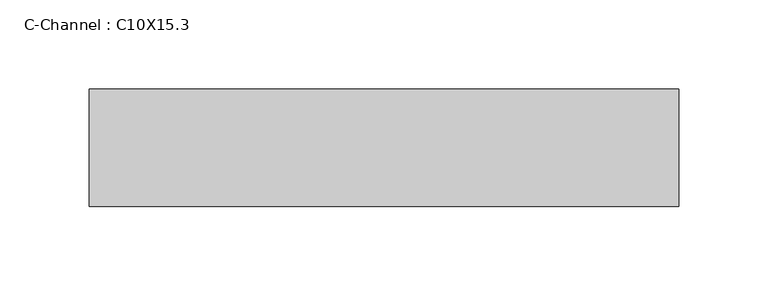
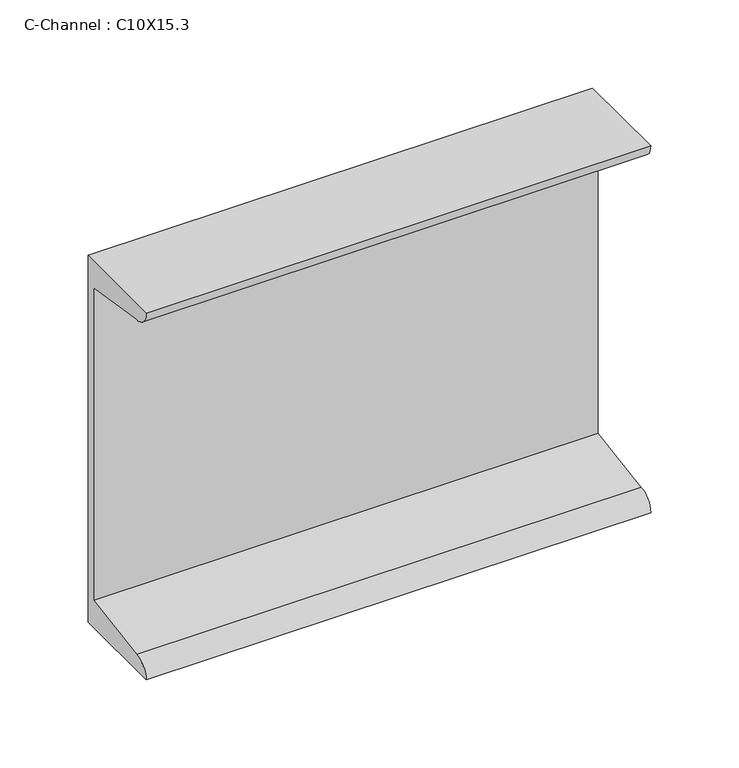
"""IFC4 building model written with IfcOpenShell, lengths in millimetres: beam geometry, C-Channel : C10X15.3."""

from ifc_helpers import new_model, si_unit, point, frame, frame_2d, origin, place, context, project, spatial, polyline, circle_curve, trimmed, segment, composite_curve, outline, extrude, source, transform, mapped, element, save


def c_channel_c10x15_3_927e855d(model_context):
    return source(origin(), model_context, "Body", "SweptSolid", [
        extrude(outline(composite_curve([segment(polyline([(16.1036, 127.0), (16.1036, -127.0), (-49.9364, -127.0)]), True, "CONTINUOUS"), segment(trimmed(circle_curve(frame_2d((-38.862, -127.0)), 11.0744), [point((-49.9364, -127.0))], [point((-38.862, -115.9256))], False, "CARTESIAN"), True, "CONTINUOUS"), segment(polyline([(-38.862, -115.9256), (10.0076, -108.1854158), (10.0076, 108.1854158), (-38.862, 115.9256)]), True, "CONTINUOUS"), segment(trimmed(circle_curve(frame_2d((-38.862, 127.0)), 11.0744), [point((-38.862, 115.9256))], [point((-49.9364, 127.0))], False, "CARTESIAN"), True, "CONTINUOUS"), segment(polyline([(-49.9364, 127.0), (16.1036, 127.0)]), True, "CONTINUOUS")], self_intersect=False)), frame((-178.308, 0.0, 0.0), z_axis=(1.0, 0.0, 0.0), x_axis=(0.0, 1.0, 0.0)), (0.0, 0.0, 1.0), 330.708),
    ])


if __name__ == "__main__":
    model = new_model("IFC4")
    model_context = context("Model", 3, world=origin())
    ifc_project = project(units=[si_unit("LENGTHUNIT", "METRE", prefix="MILLI")], contexts=[model_context])
    site = spatial("IfcSite", under=ifc_project)
    building = spatial("IfcBuilding", under=site)
    placement = place(None, origin())
    c_channel_c10x15_3_shape = c_channel_c10x15_3_927e855d(model_context)
    element("IfcBeam", 1, ObjectType="C-Channel : C10X15.3", at=placement, inside=building, context=model_context, shape_type="MappedRepresentation", body=[
        mapped(c_channel_c10x15_3_shape, transform((0.0, 0.0, 0.0), x_axis=(1.0, 0.0, 0.0), y_axis=(0.0, 1.0, 0.0), z_axis=(0.0, 0.0, 1.0))),
    ])
    save(model, "model.ifc")

# Revit data of these elements
# Type "C-Channel : C10X15.3"
#   Assembly Code = "B10"
#   W = 15.3
#   Length [instance default] = 5' - 0"
#   bf = 0' - 2.6"
#   d = 0' - 10"
#   tf = 0' - 0.436"
#   tw = 0' - 0.24"
#   x = 0' - 0.634"
#   A = 0.0311111 SF
#   Structural Material [instance default] = Steel ASTM A36
# Element 1 (IfcBeam, "C-Channel : C10X15.3")
#   Structural Material = Steel ASTM A992
#   Materials on its faces: "Steel ASTM A992"
# Materials
#   "Steel ASTM A36": class "Metal", colour RGB 199 199 199, transparency 0, Description = "Structural steel, ASTM A36 Grade B, mill finish", Cost = 0
#   "Steel ASTM A992": class "Metal", colour RGB 199 199 199, transparency 0, Description = "Structural steel 50ksi", Cost = 0
